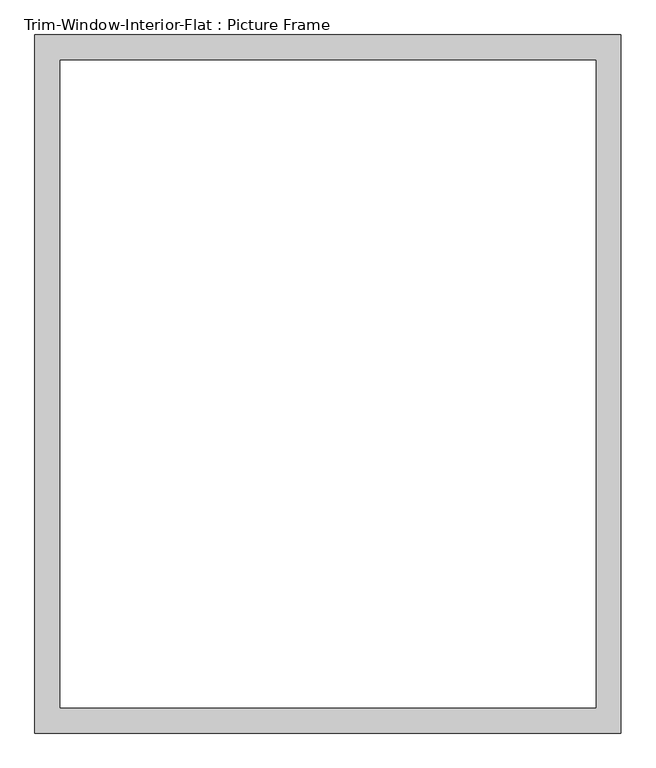
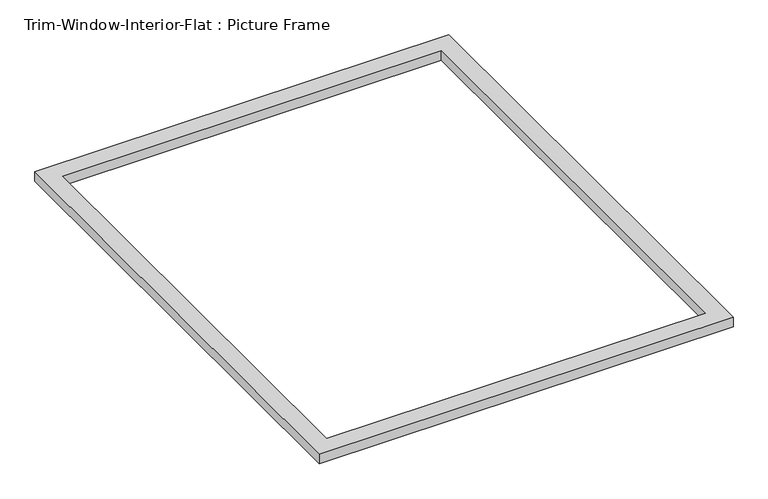
"""IFC4 building model written with IfcOpenShell, lengths in millimetres: proxy geometry, Trim-Window-Interior-Flat : Picture Frame."""

import ifcopenshell
import ifcopenshell.guid

model = None  # the IFC model being written
_history = None  # IfcOwnerHistory: only IFC2X3 demands one
_inside = {}  # id of a spatial element -> (the spatial element, [elements in it])
_under = {}  # id of a project, library or spatial element -> (it, [spatial elements below it])
_declared = {}  # id of a project -> (the project, [libraries it declares])
_typed = {}  # id of a type object -> (the type object, [elements of that type])
_made_of = {}  # id of a material, layer set ... -> (it, [elements and type objects made of it])


def new_model(schema):
    """Start an empty IFC model of exactly this schema.

    Asked for "IFC4X3", IfcOpenShell would pick the latest addendum, in which some entities
    have other attributes; the version numbers below select the first issue.
    IFC2X3 requires an IfcOwnerHistory on every rooted entity: one is made here for all.
    """
    global model, _history
    if schema == "IFC4X3":
        model = ifcopenshell.file(schema_version=(4, 3, 0, 0))
    else:
        model = ifcopenshell.file(schema=schema)
    _inside.clear()
    _under.clear()
    _declared.clear()
    _typed.clear()
    _made_of.clear()
    _history = None
    if model.schema == "IFC2X3":
        org = make("IfcOrganization", Name="unknown")
        user = make(
            "IfcPersonAndOrganization",
            ThePerson=make("IfcPerson", FamilyName="unknown"),
            TheOrganization=org,
        )
        app = make(
            "IfcApplication",
            ApplicationDeveloper=org,
            Version="unknown",
            ApplicationFullName="unknown",
            ApplicationIdentifier="unknown",
        )
        _history = make(
            "IfcOwnerHistory",
            OwningUser=user,
            OwningApplication=app,
            ChangeAction="ADDED",
            CreationDate=0,
        )
    return model


def make(cls, **values):
    """One entity of the class cls with the attributes given. An attribute that is None is left unset."""
    return model.create_entity(
        cls, **{name: value for name, value in values.items() if value is not None}
    )


def rooted(cls, **values):
    """An entity with a GlobalId (a new one), such as an element, a storey or a relation."""
    return make(cls, GlobalId=ifcopenshell.guid.new(), OwnerHistory=_history, **values)


def si_unit(unit_type, name, prefix=None):
    """IfcSIUnit, for example si_unit("LENGTHUNIT", "METRE", prefix="MILLI")."""
    return make("IfcSIUnit", UnitType=unit_type, Prefix=prefix, Name=name)


def assignment(units):
    """IfcUnitAssignment: the units of a project."""
    return None if units is None else make("IfcUnitAssignment", Units=units)


def point(xyz):
    """IfcCartesianPoint."""
    return None if xyz is None else make("IfcCartesianPoint", Coordinates=xyz)


def direction(xyz):
    """IfcDirection."""
    return None if xyz is None else make("IfcDirection", DirectionRatios=xyz)


def frame(location, z_axis=None, x_axis=None):
    """IfcAxis2Placement3D, a coordinate frame: its origin and axes. An axis left out is left unset."""
    return make(
        "IfcAxis2Placement3D",
        Location=point(location),
        Axis=direction(z_axis),
        RefDirection=direction(x_axis),
    )


def origin():
    """The frame at (0, 0, 0) with its axes left unset."""
    return frame((0.0, 0.0, 0.0))


def origin_with_axes():
    """The frame at (0, 0, 0) with the z axis (0, 0, 1) and the x axis (1, 0, 0) written out."""
    return frame((0.0, 0.0, 0.0), z_axis=(0.0, 0.0, 1.0), x_axis=(1.0, 0.0, 0.0))


def place(relative_to, where):
    """IfcLocalPlacement: puts the frame where relative to a parent placement (None: the world)."""
    return make(
        "IfcLocalPlacement", PlacementRelTo=relative_to, RelativePlacement=where
    )


def context(
    kind, dimensions, precision=None, world=None, true_north=None, identifier=None
):
    """IfcGeometricRepresentationContext, for example the 3D "Model" context."""
    return make(
        "IfcGeometricRepresentationContext",
        ContextIdentifier=identifier,
        ContextType=kind,
        CoordinateSpaceDimension=dimensions,
        Precision=precision,
        WorldCoordinateSystem=world,
        TrueNorth=true_north,
    )


def project(units=None, contexts=None):
    """IfcProject with its units and contexts."""
    return rooted(
        "IfcProject",
        Name="project",
        RepresentationContexts=contexts,
        UnitsInContext=assignment(units),
    )


def spatial(cls, under=None, at=None, **own):
    """A site, building, storey or space (cls), placed at a placement, below another one or the project."""
    s = rooted(cls, ObjectPlacement=at, **own)
    if under is not None:
        _under.setdefault(under.id(), (under, []))[1].append(s)
    return s


def polyline(points):
    """IfcPolyline through the points."""
    return make("IfcPolyline", Points=[point(p) for p in points])


def outline(outer, holes=None, kind="AREA"):
    """IfcArbitraryClosedProfileDef: a profile drawn as a closed curve; with holes, ...WithVoids."""
    if holes is None:
        return make("IfcArbitraryClosedProfileDef", ProfileType=kind, OuterCurve=outer)
    return make(
        "IfcArbitraryProfileDefWithVoids",
        ProfileType=kind,
        OuterCurve=outer,
        InnerCurves=holes,
    )


def extrude(swept, where, along, depth):
    """IfcExtrudedAreaSolid: the profile swept, set in the frame where, extruded along a direction by depth."""
    return make(
        "IfcExtrudedAreaSolid",
        SweptArea=swept,
        Position=where,
        ExtrudedDirection=direction(along),
        Depth=depth,
    )


def shape(context_of_items, identifier, shape_type, items):
    """IfcShapeRepresentation: the items that make up one representation, for example the "Body"."""
    return make(
        "IfcShapeRepresentation",
        ContextOfItems=context_of_items,
        RepresentationIdentifier=identifier,
        RepresentationType=shape_type,
        Items=items,
    )


def source(mapping_origin, context_of_items, identifier, shape_type, items):
    """IfcRepresentationMap: a shape defined once, which mapped items show again and again."""
    return make(
        "IfcRepresentationMap",
        MappingOrigin=mapping_origin,
        MappedRepresentation=shape(context_of_items, identifier, shape_type, items),
    )


def transform(
    local_origin,
    x_axis=None,
    y_axis=None,
    z_axis=None,
    scale=None,
    scale2=None,
    scale3=None,
    uniform=True,
):
    """IfcCartesianTransformationOperator3D, or its non-uniform kind. x_axis, y_axis, z_axis: its Axis1, 2, 3."""
    if uniform:
        return make(
            "IfcCartesianTransformationOperator3D",
            Axis1=direction(x_axis),
            Axis2=direction(y_axis),
            LocalOrigin=point(local_origin),
            Scale=scale,
            Axis3=direction(z_axis),
        )
    return make(
        "IfcCartesianTransformationOperator3DnonUniform",
        Axis1=direction(x_axis),
        Axis2=direction(y_axis),
        LocalOrigin=point(local_origin),
        Scale=scale,
        Axis3=direction(z_axis),
        Scale2=scale2,
        Scale3=scale3,
    )


def mapped(mapping_source, mapping_target):
    """IfcMappedItem: shows the shape of a source again, moved by a transform."""
    return make(
        "IfcMappedItem", MappingSource=mapping_source, MappingTarget=mapping_target
    )


def made_of(thing, what):
    """Note that an element or type object is made of a material, layer set ...; save() writes the relation."""
    if what is not None:
        _made_of.setdefault(what.id(), (what, []))[1].append(thing)
    return thing


def element(
    cls,
    number,
    at=None,
    inside=None,
    cuts=None,
    type_object=None,
    material=None,
    context=None,
    identifier="Body",
    shape_type=None,
    held_by="IfcProductDefinitionShape",
    body=None,
    shapes=None,
    **own,
):
    """One element of the class cls, such as IfcWall. Its Tag is "e" and its number.

    at: its placement. inside: the storey or other place that contains it. cuts: it is an
    opening in that element (IfcRelVoidsElement). A single representation is given by context,
    identifier, shape_type and body (its items); several are given by shapes. held_by: the class
    of the entity that holds the representations. save() writes the other relations.
    """
    e = rooted(cls, Tag="e%d" % number, ObjectPlacement=at, **own)
    if body is not None:
        shapes = [shape(context, identifier, shape_type, body)]
    if shapes is not None:
        e.Representation = make(held_by, Representations=shapes)
    if inside is not None:
        _inside.setdefault(inside.id(), (inside, []))[1].append(e)
    if cuts is not None:
        rooted(
            "IfcRelVoidsElement", RelatingBuildingElement=cuts, RelatedOpeningElement=e
        )
    if type_object is not None:
        _typed.setdefault(type_object.id(), (type_object, []))[1].append(e)
    return made_of(e, material)


def aggregate(whole, parts):
    """IfcRelAggregates: a whole, such as a stair, and the parts it consists of."""
    return rooted("IfcRelAggregates", RelatingObject=whole, RelatedObjects=parts)


def save(model, path):
    """Write the relations noted so far, then the file.

    IfcRelAggregates (storeys below a building ...), IfcRelContainedInSpatialStructure (elements
    in a storey), IfcRelDefinesByType, IfcRelAssociatesMaterial and IfcRelDeclares: one each for
    every whole, place, type object, material and project.
    """
    for whole, parts in _under.values():
        aggregate(whole, parts)
    for where, things in _inside.values():
        rooted(
            "IfcRelContainedInSpatialStructure",
            RelatedElements=things,
            RelatingStructure=where,
        )
    for kind, things in _typed.values():
        rooted("IfcRelDefinesByType", RelatedObjects=things, RelatingType=kind)
    for what, things in _made_of.values():
        rooted("IfcRelAssociatesMaterial", RelatedObjects=things, RelatingMaterial=what)
    for by, libraries in _declared.values():
        rooted("IfcRelDeclares", RelatingContext=by, RelatedDefinitions=libraries)
    model.write(path)


def trim_window_interior_flat_picture_frame_691deff5(model_context):
    return source(origin(), model_context, "Body", "SweptSolid", [
        extrude(outline(polyline([(666.75, 44.45), (666.75, -1543.05), (-666.75, -1543.05), (-666.75, 44.45), (666.75, 44.45)]), holes=[polyline([(609.6, -12.7), (-609.6, -12.7), (-609.6, -1485.9), (609.6, -1485.9), (609.6, -12.7)])]), origin_with_axes(), (0.0, 0.0, 1.0), 31.75),
    ])


if __name__ == "__main__":
    model = new_model("IFC4")
    model_context = context("Model", 3, world=origin())
    ifc_project = project(units=[si_unit("LENGTHUNIT", "METRE", prefix="MILLI")], contexts=[model_context])
    site = spatial("IfcSite", under=ifc_project)
    building = spatial("IfcBuilding", under=site)
    placement = place(None, origin())
    trim_window_interior_flat_picture_frame_shape = trim_window_interior_flat_picture_frame_691deff5(model_context)
    element("IfcBuildingElementProxy", 1, Name="Trim-Window-Interior-Flat : Picture Frame", ObjectType="Trim-Window-Interior-Flat : Picture Frame", at=placement, inside=building, context=model_context, shape_type="MappedRepresentation", body=[
        mapped(trim_window_interior_flat_picture_frame_shape, transform((0.0, 0.0, 0.0), x_axis=(1.0, 0.0, 0.0), y_axis=(0.0, 1.0, 0.0), z_axis=(0.0, 0.0, 1.0))),
    ])
    save(model, "model.ifc")

# Revit data of these elements
# Type "Trim-Window-Interior-Flat : Picture Frame"
#   Trim Thickness_Picture Frame = 0' - 1 1/4"
#   Trim Width = 0' - 2 1/4"
#   Trim Thickness_with Sill = 0' - 0 3/4"
#   Sill Thickness = 0' - 1 1/4"
#   Opening Width [instance default] = 2' - 0"
#   Opening Height [instance default] = 3' - 0"
#   Default Elevation = 4' - 0"
#   Sill = no
#   Picture Frame = yes
#   Trim Material [instance default] = none
# Element 1 (IfcBuildingElementProxy, "Trim-Window-Interior-Flat : Picture Frame")
#   Opening Width = 4' - 1"
#   Opening Height = 4' - 11"
#   Trim Material = Wood - Stained
#   Materials on its faces: "Wood - Stained"
# Materials
#   "Wood - Stained": class "Wood", colour RGB 224 178 126, transparency 0, Cost = 0
